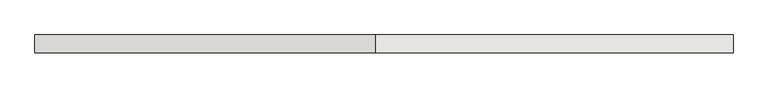
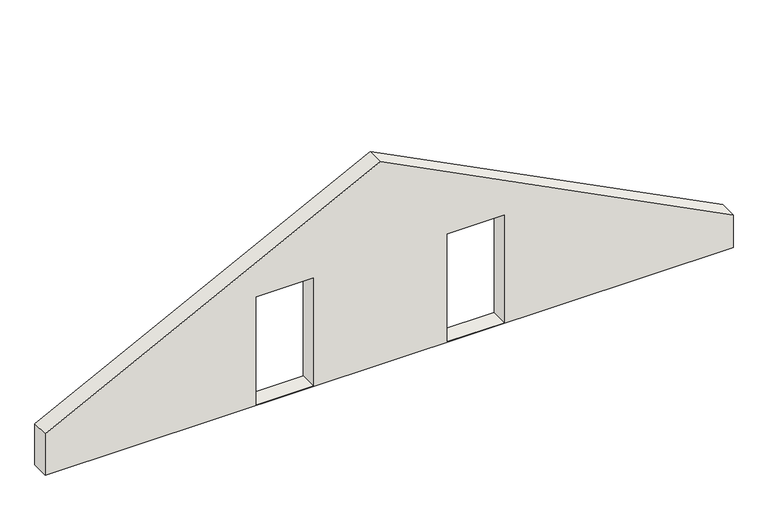
"""IFC4 building model written with IfcOpenShell, lengths in millimetres: wall geometry, 0_3d."""

from ifc_helpers import new_model, si_unit, frame, origin, place, context, project, spatial, polyline, outline, extrude, source, transform, mapped, element, save


def wall_b6a05950(model_context):
    return source(origin(), model_context, "Body", "SweptSolid", [
        extrude(outline(polyline([(4251.6781465, 6650.0), (863.3339073, 0.0), (0.0, 0.0), (0.0, 13650.0), (685.0, 13650.0), (4251.6781465, 6650.0)]), holes=[polyline([(10.0, 4190.0), (2270.0, 4190.0), (2270.0, 5325.0), (10.0, 5325.0), (10.0, 4190.0)]), polyline([(10.0, 7975.0), (2270.0, 7975.0), (2270.0, 9110.0), (10.0, 9110.0), (10.0, 7975.0)])]), frame((0.0, 0.0, 0.0), z_axis=(0.0, 1.0, 0.0), x_axis=(0.0, 0.0, 1.0)), (0.0, 0.0, 1.0), 350.0),
    ])


if __name__ == "__main__":
    model = new_model("IFC4")
    model_context = context("Model", 3, world=origin())
    ifc_project = project(units=[si_unit("LENGTHUNIT", "METRE", prefix="MILLI")], contexts=[model_context])
    site = spatial("IfcSite", under=ifc_project)
    building = spatial("IfcBuilding", under=site)
    placement = place(None, origin())
    wall_shape = wall_b6a05950(model_context)
    element("IfcWall", 1, ObjectType="0_3d", at=placement, inside=building, context=model_context, shape_type="MappedRepresentation", body=[
        mapped(wall_shape, transform((0.0, 0.0, 0.0), x_axis=(1.0, 0.0, 0.0), y_axis=(0.0, 1.0, 0.0), z_axis=(0.0, 0.0, 1.0))),
    ])
    save(model, "model.ifc")

# Revit data of these elements
# Element 1 (IfcWall, "0_3d")
#   Materials on its faces: "holzschalung"
# Materials
#   "holzschalung": class "Unassigned", colour RGB 128 128 128, transparency 0
